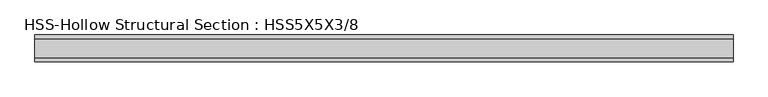
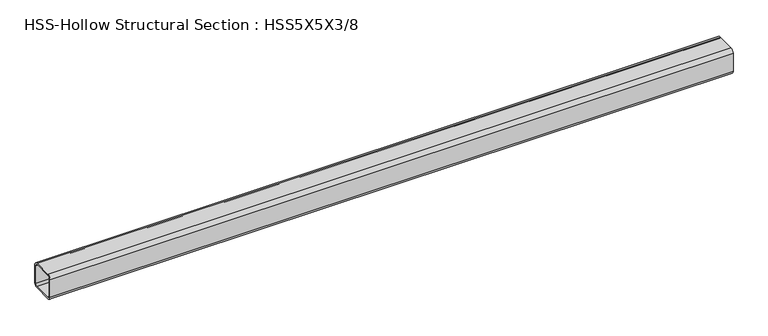
"""IFC4 building model written with IfcOpenShell, lengths in millimetres: member geometry, HSS-Hollow Structural Section : HSS5X5X3/8."""

from ifc_helpers import new_model, si_unit, point, frame, frame_2d, origin, place, context, project, spatial, polyline, circle_curve, trimmed, segment, composite_curve, outline, extrude, source, transform, mapped, element, save


def hss_hollow_structural_section_hss5x5x3_8_017cef90(model_context):
    return source(origin(), model_context, "Body", "SweptSolid", [
        extrude(outline(composite_curve([segment(polyline([(63.5, 45.7708), (63.5, -45.7708)]), True, "CONTINUOUS"), segment(trimmed(circle_curve(frame_2d((45.7708, -45.7708)), 17.7292), [point((63.5, -45.7708))], [point((45.7708, -63.5))], False, "CARTESIAN"), True, "CONTINUOUS"), segment(polyline([(45.7708, -63.5), (-45.7708, -63.5)]), True, "CONTINUOUS"), segment(trimmed(circle_curve(frame_2d((-45.7708, -45.7708)), 17.7292), [point((-45.7708, -63.5))], [point((-63.5, -45.7708))], False, "CARTESIAN"), True, "CONTINUOUS"), segment(polyline([(-63.5, -45.7708), (-63.5, 45.7708)]), True, "CONTINUOUS"), segment(trimmed(circle_curve(frame_2d((-45.7708, 45.7708)), 17.7292), [point((-63.5, 45.7708))], [point((-45.7708, 63.5))], False, "CARTESIAN"), True, "CONTINUOUS"), segment(polyline([(-45.7708, 63.5), (45.7708, 63.5)]), True, "CONTINUOUS"), segment(trimmed(circle_curve(frame_2d((45.7708, 45.7708)), 17.7292), [point((45.7708, 63.5))], [point((63.5, 45.7708))], False, "CARTESIAN"), True, "CONTINUOUS")], self_intersect=False), holes=[composite_curve([segment(trimmed(circle_curve(frame_2d((-45.7708, 45.7708)), 8.8646), [point((-45.7708, 54.6354))], [point((-54.6354, 45.7708))], True, "CARTESIAN"), True, "CONTINUOUS"), segment(polyline([(-54.6354, 45.7708), (-54.6354, -45.7708)]), True, "CONTINUOUS"), segment(trimmed(circle_curve(frame_2d((-45.7708, -45.7708)), 8.8646), [point((-54.6354, -45.7708))], [point((-45.7708, -54.6354))], True, "CARTESIAN"), True, "CONTINUOUS"), segment(polyline([(-45.7708, -54.6354), (45.7708, -54.6354)]), True, "CONTINUOUS"), segment(trimmed(circle_curve(frame_2d((45.7708, -45.7708)), 8.8646), [point((45.7708, -54.6354))], [point((54.6354, -45.7708))], True, "CARTESIAN"), True, "CONTINUOUS"), segment(polyline([(54.6354, -45.7708), (54.6354, 45.7708)]), True, "CONTINUOUS"), segment(trimmed(circle_curve(frame_2d((45.7708, 45.7708)), 8.8646), [point((54.6354, 45.7708))], [point((45.7708, 54.6354))], True, "CARTESIAN"), True, "CONTINUOUS"), segment(polyline([(45.7708, 54.6354), (-45.7708, 54.6354)]), True, "CONTINUOUS")], self_intersect=False)]), frame((-1660.5512918, 0.0, 0.0), z_axis=(1.0, 0.0, 0.0), x_axis=(0.0, 1.0, 0.0)), (0.0, 0.0, 1.0), 3321.1025836),
    ])


if __name__ == "__main__":
    model = new_model("IFC4")
    model_context = context("Model", 3, world=origin())
    ifc_project = project(units=[si_unit("LENGTHUNIT", "METRE", prefix="MILLI")], contexts=[model_context])
    site = spatial("IfcSite", under=ifc_project)
    building = spatial("IfcBuilding", under=site)
    placement = place(None, origin())
    hss_hollow_structural_section_hss5x5x3_8_shape = hss_hollow_structural_section_hss5x5x3_8_017cef90(model_context)
    element("IfcMember", 1, ObjectType="HSS-Hollow Structural Section : HSS5X5X3/8", at=placement, inside=building, context=model_context, shape_type="MappedRepresentation", body=[
        mapped(hss_hollow_structural_section_hss5x5x3_8_shape, transform((0.0, 0.0, 0.0), x_axis=(1.0, 0.0, 0.0), y_axis=(0.0, 1.0, 0.0), z_axis=(0.0, 0.0, 1.0))),
    ])
    save(model, "model.ifc")

# Revit data of these elements
# Project information
#   TBC Electrician = "ELECTRICIAN HERE"
#   TBC Fire Protection = "FP HERE"
#   TBC Plumber = "PLUMBER HERE"
#   TBC HVAC = "HVAC HERE"
#   TBC Other Company 1 = "MISC COMPANY 1"
#   TBC Other Company 2 = "MISC COMPANY 2"
#   TBC COORDINATOR = "NAME OF VCC"
#   Project Issue Date = "2010.12.07"
#   Project Status = "Project Status"
#   Client Name = "Owner"
#   Project Address = "111 BOYLSTON STREET, \nBROOKLINE MA"
#   Project Name = "HOMEWOOD SUITES"
#   Project Number = "13381"
# Type "HSS-Hollow Structural Section : HSS5X5X3/8"
#   Assembly Code = "B10"
#   Shape = "Square"
#   W = 22.3
#   Ht = 0' - 5"
#   Length [instance default] = 5' - 0"
#   b = 0' - 5"
#   kr = 0' - 0.698"
#   t = 0' - 0.349"
#   A = 0.0429167 SF
#   Structural Material [instance default] = Steel ASTM A500, Grade B, Rectangular and Square
# Element 1 (IfcMember, "HSS-Hollow Structural Section : HSS5X5X3/8")
#   Materials on its faces: "Steel ASTM A500, Grade B, Rectangular and Square"
# Materials
#   "Steel ASTM A500, Grade B, Rectangular and Square": class "Metal", colour RGB 199 199 199, transparency 0, Description = "Carbon steel", Cost = 0
